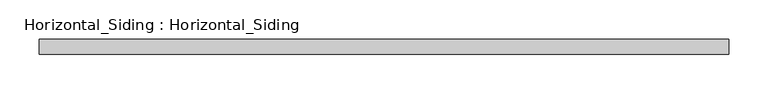
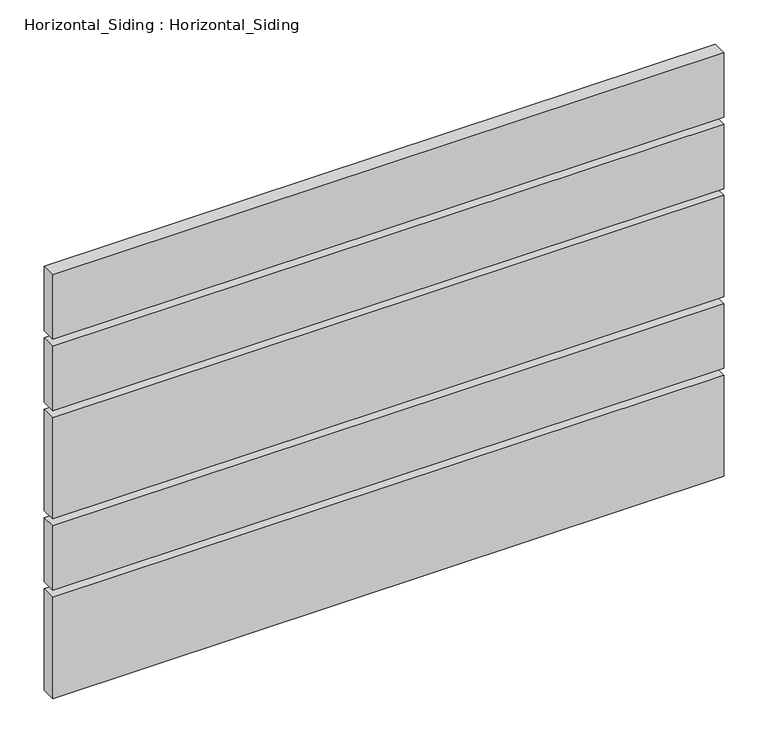
"""IFC4 building model written with IfcOpenShell, lengths in millimetres: plate geometry, Horizontal_Siding : Horizontal_Siding."""

import ifcopenshell
import ifcopenshell.guid

model = None  # the IFC model being written
_history = None  # IfcOwnerHistory: only IFC2X3 demands one
_inside = {}  # id of a spatial element -> (the spatial element, [elements in it])
_under = {}  # id of a project, library or spatial element -> (it, [spatial elements below it])
_declared = {}  # id of a project -> (the project, [libraries it declares])
_typed = {}  # id of a type object -> (the type object, [elements of that type])
_made_of = {}  # id of a material, layer set ... -> (it, [elements and type objects made of it])


def new_model(schema):
    """Start an empty IFC model of exactly this schema.

    Asked for "IFC4X3", IfcOpenShell would pick the latest addendum, in which some entities
    have other attributes; the version numbers below select the first issue.
    IFC2X3 requires an IfcOwnerHistory on every rooted entity: one is made here for all.
    """
    global model, _history
    if schema == "IFC4X3":
        model = ifcopenshell.file(schema_version=(4, 3, 0, 0))
    else:
        model = ifcopenshell.file(schema=schema)
    _inside.clear()
    _under.clear()
    _declared.clear()
    _typed.clear()
    _made_of.clear()
    _history = None
    if model.schema == "IFC2X3":
        org = make("IfcOrganization", Name="unknown")
        user = make(
            "IfcPersonAndOrganization",
            ThePerson=make("IfcPerson", FamilyName="unknown"),
            TheOrganization=org,
        )
        app = make(
            "IfcApplication",
            ApplicationDeveloper=org,
            Version="unknown",
            ApplicationFullName="unknown",
            ApplicationIdentifier="unknown",
        )
        _history = make(
            "IfcOwnerHistory",
            OwningUser=user,
            OwningApplication=app,
            ChangeAction="ADDED",
            CreationDate=0,
        )
    return model


def make(cls, **values):
    """One entity of the class cls with the attributes given. An attribute that is None is left unset."""
    return model.create_entity(
        cls, **{name: value for name, value in values.items() if value is not None}
    )


def rooted(cls, **values):
    """An entity with a GlobalId (a new one), such as an element, a storey or a relation."""
    return make(cls, GlobalId=ifcopenshell.guid.new(), OwnerHistory=_history, **values)


def si_unit(unit_type, name, prefix=None):
    """IfcSIUnit, for example si_unit("LENGTHUNIT", "METRE", prefix="MILLI")."""
    return make("IfcSIUnit", UnitType=unit_type, Prefix=prefix, Name=name)


def assignment(units):
    """IfcUnitAssignment: the units of a project."""
    return None if units is None else make("IfcUnitAssignment", Units=units)


def point(xyz):
    """IfcCartesianPoint."""
    return None if xyz is None else make("IfcCartesianPoint", Coordinates=xyz)


def direction(xyz):
    """IfcDirection."""
    return None if xyz is None else make("IfcDirection", DirectionRatios=xyz)


def frame(location, z_axis=None, x_axis=None):
    """IfcAxis2Placement3D, a coordinate frame: its origin and axes. An axis left out is left unset."""
    return make(
        "IfcAxis2Placement3D",
        Location=point(location),
        Axis=direction(z_axis),
        RefDirection=direction(x_axis),
    )


def origin():
    """The frame at (0, 0, 0) with its axes left unset."""
    return frame((0.0, 0.0, 0.0))


def place(relative_to, where):
    """IfcLocalPlacement: puts the frame where relative to a parent placement (None: the world)."""
    return make(
        "IfcLocalPlacement", PlacementRelTo=relative_to, RelativePlacement=where
    )


def context(
    kind, dimensions, precision=None, world=None, true_north=None, identifier=None
):
    """IfcGeometricRepresentationContext, for example the 3D "Model" context."""
    return make(
        "IfcGeometricRepresentationContext",
        ContextIdentifier=identifier,
        ContextType=kind,
        CoordinateSpaceDimension=dimensions,
        Precision=precision,
        WorldCoordinateSystem=world,
        TrueNorth=true_north,
    )


def project(units=None, contexts=None):
    """IfcProject with its units and contexts."""
    return rooted(
        "IfcProject",
        Name="project",
        RepresentationContexts=contexts,
        UnitsInContext=assignment(units),
    )


def spatial(cls, under=None, at=None, **own):
    """A site, building, storey or space (cls), placed at a placement, below another one or the project."""
    s = rooted(cls, ObjectPlacement=at, **own)
    if under is not None:
        _under.setdefault(under.id(), (under, []))[1].append(s)
    return s


def polyline(points):
    """IfcPolyline through the points."""
    return make("IfcPolyline", Points=[point(p) for p in points])


def outline(outer, holes=None, kind="AREA"):
    """IfcArbitraryClosedProfileDef: a profile drawn as a closed curve; with holes, ...WithVoids."""
    if holes is None:
        return make("IfcArbitraryClosedProfileDef", ProfileType=kind, OuterCurve=outer)
    return make(
        "IfcArbitraryProfileDefWithVoids",
        ProfileType=kind,
        OuterCurve=outer,
        InnerCurves=holes,
    )


def extrude(swept, where, along, depth):
    """IfcExtrudedAreaSolid: the profile swept, set in the frame where, extruded along a direction by depth."""
    return make(
        "IfcExtrudedAreaSolid",
        SweptArea=swept,
        Position=where,
        ExtrudedDirection=direction(along),
        Depth=depth,
    )


def shape(context_of_items, identifier, shape_type, items):
    """IfcShapeRepresentation: the items that make up one representation, for example the "Body"."""
    return make(
        "IfcShapeRepresentation",
        ContextOfItems=context_of_items,
        RepresentationIdentifier=identifier,
        RepresentationType=shape_type,
        Items=items,
    )


def source(mapping_origin, context_of_items, identifier, shape_type, items):
    """IfcRepresentationMap: a shape defined once, which mapped items show again and again."""
    return make(
        "IfcRepresentationMap",
        MappingOrigin=mapping_origin,
        MappedRepresentation=shape(context_of_items, identifier, shape_type, items),
    )


def transform(
    local_origin,
    x_axis=None,
    y_axis=None,
    z_axis=None,
    scale=None,
    scale2=None,
    scale3=None,
    uniform=True,
):
    """IfcCartesianTransformationOperator3D, or its non-uniform kind. x_axis, y_axis, z_axis: its Axis1, 2, 3."""
    if uniform:
        return make(
            "IfcCartesianTransformationOperator3D",
            Axis1=direction(x_axis),
            Axis2=direction(y_axis),
            LocalOrigin=point(local_origin),
            Scale=scale,
            Axis3=direction(z_axis),
        )
    return make(
        "IfcCartesianTransformationOperator3DnonUniform",
        Axis1=direction(x_axis),
        Axis2=direction(y_axis),
        LocalOrigin=point(local_origin),
        Scale=scale,
        Axis3=direction(z_axis),
        Scale2=scale2,
        Scale3=scale3,
    )


def mapped(mapping_source, mapping_target):
    """IfcMappedItem: shows the shape of a source again, moved by a transform."""
    return make(
        "IfcMappedItem", MappingSource=mapping_source, MappingTarget=mapping_target
    )


def made_of(thing, what):
    """Note that an element or type object is made of a material, layer set ...; save() writes the relation."""
    if what is not None:
        _made_of.setdefault(what.id(), (what, []))[1].append(thing)
    return thing


def element(
    cls,
    number,
    at=None,
    inside=None,
    cuts=None,
    type_object=None,
    material=None,
    context=None,
    identifier="Body",
    shape_type=None,
    held_by="IfcProductDefinitionShape",
    body=None,
    shapes=None,
    **own,
):
    """One element of the class cls, such as IfcWall. Its Tag is "e" and its number.

    at: its placement. inside: the storey or other place that contains it. cuts: it is an
    opening in that element (IfcRelVoidsElement). A single representation is given by context,
    identifier, shape_type and body (its items); several are given by shapes. held_by: the class
    of the entity that holds the representations. save() writes the other relations.
    """
    e = rooted(cls, Tag="e%d" % number, ObjectPlacement=at, **own)
    if body is not None:
        shapes = [shape(context, identifier, shape_type, body)]
    if shapes is not None:
        e.Representation = make(held_by, Representations=shapes)
    if inside is not None:
        _inside.setdefault(inside.id(), (inside, []))[1].append(e)
    if cuts is not None:
        rooted(
            "IfcRelVoidsElement", RelatingBuildingElement=cuts, RelatedOpeningElement=e
        )
    if type_object is not None:
        _typed.setdefault(type_object.id(), (type_object, []))[1].append(e)
    return made_of(e, material)


def aggregate(whole, parts):
    """IfcRelAggregates: a whole, such as a stair, and the parts it consists of."""
    return rooted("IfcRelAggregates", RelatingObject=whole, RelatedObjects=parts)


def save(model, path):
    """Write the relations noted so far, then the file.

    IfcRelAggregates (storeys below a building ...), IfcRelContainedInSpatialStructure (elements
    in a storey), IfcRelDefinesByType, IfcRelAssociatesMaterial and IfcRelDeclares: one each for
    every whole, place, type object, material and project.
    """
    for whole, parts in _under.values():
        aggregate(whole, parts)
    for where, things in _inside.values():
        rooted(
            "IfcRelContainedInSpatialStructure",
            RelatedElements=things,
            RelatingStructure=where,
        )
    for kind, things in _typed.values():
        rooted("IfcRelDefinesByType", RelatedObjects=things, RelatingType=kind)
    for what, things in _made_of.values():
        rooted("IfcRelAssociatesMaterial", RelatedObjects=things, RelatingMaterial=what)
    for by, libraries in _declared.values():
        rooted("IfcRelDeclares", RelatingContext=by, RelatedDefinitions=libraries)
    model.write(path)


def horizontal_siding_horizontal_siding_750e89fe(model_context):
    return source(origin(), model_context, "Body", "SweptSolid", [
        extrude(outline(polyline([(437.5115389, -19.05), (-437.5115389, -19.05), (-437.5115389, 0.0), (437.5115389, 0.0), (437.5115389, -19.05)])), frame((0.0, 0.0, 9.525), z_axis=(0.0, 0.0, 1.0), x_axis=(1.0, 0.0, 0.0)), (0.0, 0.0, 1.0), 139.7),
        extrude(outline(polyline([(437.5115389, -19.05), (-437.5115389, -19.05), (-437.5115389, 0.0), (437.5115389, 0.0), (437.5115389, -19.05)])), frame((0.0, 0.0, 158.75), z_axis=(0.0, 0.0, 1.0), x_axis=(1.0, 0.0, 0.0)), (0.0, 0.0, 1.0), 88.9),
        extrude(outline(polyline([(437.5115389, -19.05), (-437.5115389, -19.05), (-437.5115389, 0.0), (437.5115389, 0.0), (437.5115389, -19.05)])), frame((0.0, 0.0, 257.175), z_axis=(0.0, 0.0, 1.0), x_axis=(1.0, 0.0, 0.0)), (0.0, 0.0, 1.0), 139.7),
        extrude(outline(polyline([(437.5115389, -19.05), (-437.5115389, -19.05), (-437.5115389, 0.0), (437.5115389, 0.0), (437.5115389, -19.05)])), frame((0.0, 0.0, 406.4), z_axis=(0.0, 0.0, 1.0), x_axis=(1.0, 0.0, 0.0)), (0.0, 0.0, 1.0), 88.9),
        extrude(outline(polyline([(437.5115389, -19.05), (-437.5115389, -19.05), (-437.5115389, 0.0), (437.5115389, 0.0), (437.5115389, -19.05)])), frame((0.0, 0.0, 504.825), z_axis=(0.0, 0.0, 1.0), x_axis=(1.0, 0.0, 0.0)), (0.0, 0.0, 1.0), 88.9),
    ])


if __name__ == "__main__":
    model = new_model("IFC4")
    model_context = context("Model", 3, world=origin())
    ifc_project = project(units=[si_unit("LENGTHUNIT", "METRE", prefix="MILLI")], contexts=[model_context])
    site = spatial("IfcSite", under=ifc_project)
    building = spatial("IfcBuilding", under=site)
    placement = place(None, origin())
    horizontal_siding_horizontal_siding_shape = horizontal_siding_horizontal_siding_750e89fe(model_context)
    element("IfcPlate", 1, ObjectType="Horizontal_Siding : Horizontal_Siding", at=placement, inside=building, context=model_context, shape_type="MappedRepresentation", body=[
        mapped(horizontal_siding_horizontal_siding_shape, transform((0.0, 0.0, 0.0), x_axis=(1.0, 0.0, 0.0), y_axis=(0.0, 1.0, 0.0), z_axis=(0.0, 0.0, 1.0))),
    ])
    save(model, "model.ifc")

# Revit data of these elements
# Type "Horizontal_Siding : Horizontal_Siding"
#   Analytic Construction = "<None>"
#   extend = 0' - 2 3/4"
#   Width_2 = 0' - 3 1/2"
#   Width_1 = 0' - 5 1/2"
#   Gap = 0' - 0 3/8"
#   Plank Material = SLOTTED WOOD FENCE (THERMALLY MODIFIED WOOD: ARBOR WOOD)\n(EXTERIOR STAIN : PENOFIN VERDE EXT. STAIN - COLOR: CEDAR)
# Element 1 (IfcPlate, "Horizontal_Siding : Horizontal_Siding")
#   Materials on its faces: "SLOTTED WOOD FENCE (THERMALLY MODIFIED WOOD: ARBOR WOOD)\n(EXTERIOR STAIN : PENOFIN VERDE EXT. STAIN - COLOR: CEDAR)"
# Materials
#   "SLOTTED WOOD FENCE (THERMALLY MODIFIED WOOD: ARBOR WOOD)\n(EXTERIOR STAIN : PENOFIN VERDE EXT. STAIN - COLOR: CEDAR)": class "Wood", colour RGB 164 134 123, transparency 0, Description = "Pinus Echinata", Cost = 0
